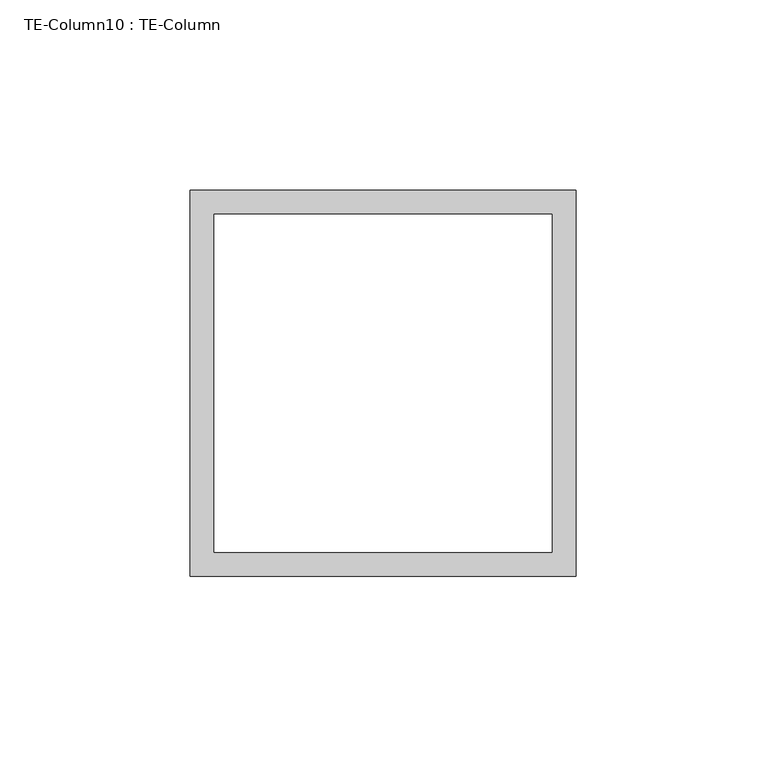
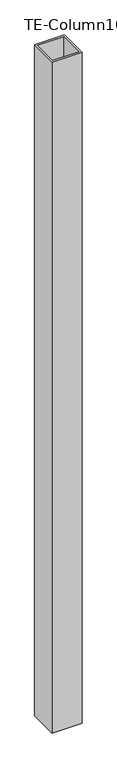
"""IFC4 building model written with IfcOpenShell, lengths in millimetres: proxy geometry, TE-Column10 : TE-Column."""

from ifc_helpers import new_model, si_unit, frame, origin, place, context, project, spatial, polyline, outline, extrude, source, transform, mapped, element, save


def te_column10_te_column_7b45b3bc(model_context):
    return source(origin(), model_context, "Body", "SweptSolid", [
        extrude(outline(polyline([(587467.4934739, -531667.7913841), (587467.4934739, -531769.3913841), (587365.8934739, -531769.3913841), (587365.8934739, -531667.7913841), (587467.4934739, -531667.7913841)]), holes=[polyline([(587372.2434739, -531674.1413841), (587372.2434739, -531763.0413841), (587461.1434739, -531763.0413841), (587461.1434739, -531674.1413841), (587372.2434739, -531674.1413841)])]), frame((0.0, 0.0, 28.575), z_axis=(0.0, 0.0, 1.0), x_axis=(1.0, 0.0, 0.0)), (0.0, 0.0, 1.0), 2406.65),
    ])


if __name__ == "__main__":
    model = new_model("IFC4")
    model_context = context("Model", 3, world=origin())
    ifc_project = project(units=[si_unit("LENGTHUNIT", "METRE", prefix="MILLI")], contexts=[model_context])
    site = spatial("IfcSite", under=ifc_project)
    building = spatial("IfcBuilding", under=site)
    placement = place(None, origin())
    te_column10_te_column_shape = te_column10_te_column_7b45b3bc(model_context)
    element("IfcBuildingElementProxy", 1, Name="TE-Column10 : TE-Column", ObjectType="TE-Column10 : TE-Column", at=placement, inside=building, context=model_context, shape_type="MappedRepresentation", body=[
        mapped(te_column10_te_column_shape, transform((0.0, 0.0, 0.0), x_axis=(1.0, 0.0, 0.0), y_axis=(0.0, 1.0, 0.0), z_axis=(0.0, 0.0, 1.0))),
    ])
    save(model, "model.ifc")

# Revit data of these elements
# Element 1 (IfcBuildingElementProxy, "TE-Column10 : TE-Column")
#   Materials on its faces: "4\"X4\" GALV. HSS TUBING"
# Materials
#   "4\"X4\" GALV. HSS TUBING": class "Generic", colour RGB 211 211 207, transparency 0, Cost = 0
